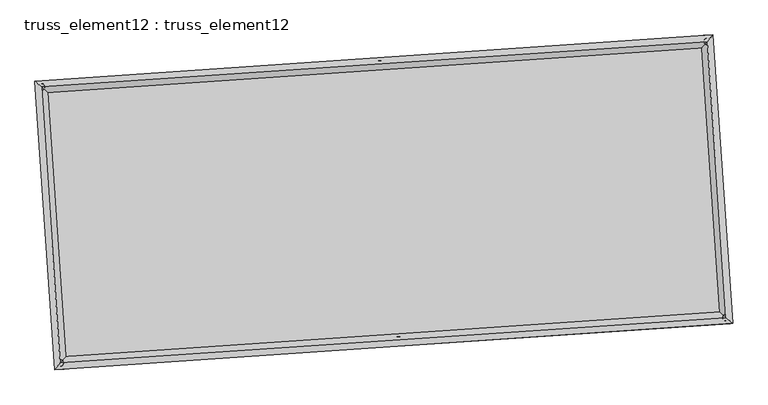
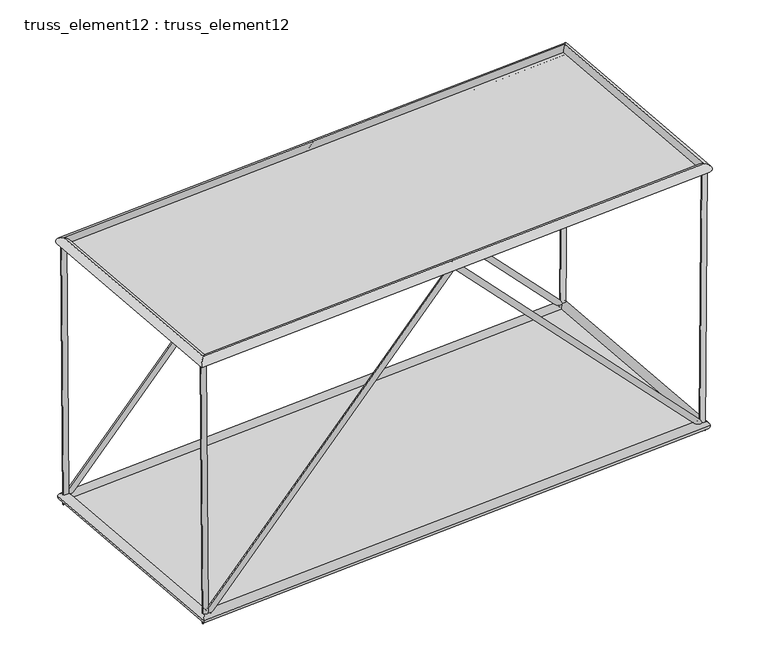
"""IFC4 building model written with IfcOpenShell, lengths in millimetres: plate geometry, truss_element12 : truss_element12."""

from ifc_helpers import new_model, si_unit, frame, origin, origin_with_axes, place, context, project, spatial, polyline, circle_curve, ellipse_curve, outline, extrude, source, transform, mapped, element, save
from ifc_brep_helpers import plane_surface, cylinder_surface, advanced_brep


def truss_element12_truss_element12_81932074(model_context):
    return source(origin(), model_context, "Body", "SolidModel", [
        advanced_brep(
        [(-3702.688172, 2273.6501932, 5000.2343714), (-3801.788684, 2260.2891126, 4999.4793629), (-3665.8706913, 2276.1606372, 123.2387715), (-3763.1161915, 2262.9260429, -123.2387715), (1063.4172149, 2598.6328018, 5071.9820194), (1063.8699312, 2592.0598775, 4927.7362286), (5793.2948238, 2921.145176, 123.2430249), (5891.4661532, 2921.2353125, -123.2430249), (5829.5270694, 2923.6157151, 5000.2328852), (5929.5240788, 2923.8303377, 4999.4898764)],
        [
            (0, 1, circle_curve(frame((-3752.238428, 2266.9696529, 4999.8568672), z_axis=(-0.007548997314577087, -0.000514737430455595, 0.999971373432721), x_axis=(-0.13361086689497337, 0.9910337470163174, -0.0004985201818760374)), 50.0)),
            (1, 0, circle_curve(frame((-3752.238428, 2266.9696529, 4999.8568672), z_axis=(-0.007548997314577087, -0.000514737430455595, 0.999971373432721), x_axis=(-0.13361086689497337, 0.9910337470163174, -0.0004985201818760374)), 50.0)),
            (0, 2),
            (2, 3, ellipse_curve(frame((-3714.4934414, 2269.54334, 0.0), z_axis=(-0.9271929359308112, -0.06322176171080186, 0.36921033084975474), x_axis=(0.36835501674811216, 0.025116728343544507, 0.9293458622029878)), 132.8968359, 50.0)),
            (3, 1),
            (3, 2, ellipse_curve(frame((-3714.4934414, 2269.54334, 0.0), z_axis=(-0.9271929359308112, -0.06322176171080186, 0.36921033084975474), x_axis=(0.36835501674811216, 0.025116728343544507, 0.9293458622029878)), 132.8968359, 50.0)),
            (2, 4),
            (4, 5, ellipse_curve(frame((1063.6435731, 2595.3463397, 4999.859124), z_axis=(-0.9976833955843888, -0.06802823819525586, -3.135687396447292e-05), x_axis=(3.12842325072798e-05, 2.133152891987861e-06, -0.9999999995083733)), 72.2799434, 50.0)),
            (5, 3),
            (5, 4, ellipse_curve(frame((1063.6435731, 2595.3463397, 4999.859124), z_axis=(-0.9976833955843888, -0.06802823819525586, -3.135687396447292e-05), x_axis=(3.12842325072798e-05, 2.133152891987861e-06, -0.9999999995083733)), 72.2799434, 50.0)),
            (4, 6),
            (6, 7, ellipse_curve(frame((5842.3804885, 2921.1902443, 0.0), z_axis=(-0.9271592320010842, -0.06321946356795421, -0.36929535326258833), x_axis=(-0.36843984219769044, -0.025122512268499313, 0.9293120800133075)), 132.9062538, 50.0)),
            (7, 5),
            (7, 6, ellipse_curve(frame((5842.3804885, 2921.1902443, 0.0), z_axis=(-0.9271592320010842, -0.06321946356795421, -0.36929535326258833), x_axis=(-0.36843984219769044, -0.025122512268499313, 0.9293120800133075)), 132.9062538, 50.0)),
            (8, 9, circle_curve(frame((5879.5255741, 2923.7230264, 4999.8613808), z_axis=(0.007429017120522426, 0.0005065564371105527, 0.9999722761682942), x_axis=(-0.0021499302803911083, 0.999997568554261, -0.0004905969378120464)), 50.0)),
            (9, 8, circle_curve(frame((5879.5255741, 2923.7230264, 4999.8613808), z_axis=(0.007429017120522426, 0.0005065564371105527, 0.9999722761682942), x_axis=(-0.0021499302803911083, 0.999997568554261, -0.0004905969378120464)), 50.0)),
            (6, 8),
            (9, 7),
        ],
        [
            plane_surface(frame((-3752.238428, 2316.9696463, 4999.8826048), z_axis=(-0.007548997314575647, -0.0005147374304560255, 0.9999713734327211), x_axis=(0.9999715059138159, -3.885862204455747e-06, 0.007548996314447718))),
            cylinder_surface(frame((-3752.238428, 2266.9696529, 4999.8568672), z_axis=(-0.007548997314577087, -0.000514737430455595, 0.999971373432721), x_axis=(-0.13361086689497337, 0.9910337470163174, -0.0004985201818760374)), 50.0),
            cylinder_surface(frame((-3714.4934414, 2269.54334, 0.0), z_axis=(-0.6901297168790946, -0.04705732196532738, -0.7221541264368931), x_axis=(-0.02041156189161515, 0.9987523773136525, -0.04557474027871566)), 50.0),
            cylinder_surface(frame((1063.6435731, 2595.3463397, 4999.859124), z_axis=(-0.6901748995971223, -0.04706040280311382, 0.7221107438988223), x_axis=(-0.115346442987764, 0.9922791286529746, -0.04557772405203943)), 50.0),
            plane_surface(frame((5879.5255741, 2873.7230329, 4999.8867094), z_axis=(0.007429017120522355, 0.0005065564371127904, 0.9999722761682942), x_axis=(0.999972404471555, -3.7633202953912764e-06, -0.0074290161673289294))),
            cylinder_surface(frame((5842.3804885, 2921.1902443, 0.0), z_axis=(-0.007429017120522424, -0.0005065564371105526, -0.999972276168294), x_axis=(-0.0021499302803911083, 0.999997568554261, -0.0004905969378120464)), 50.0),
        ],
        [
            (0, [[1, 2]]),
            (1, [[-1, 3, 4, 5]]),
            (1, [[-2, -5, 6, -3]]),
            (2, [[-4, 7, 8, 9]]),
            (2, [[-6, -9, 10, -7]]),
            (3, [[-8, 11, 12, 13]]),
            (3, [[-10, -13, 14, -11]]),
            (4, [[15, 16]]),
            (5, [[-12, 17, -16, 18]]),
            (5, [[-14, -18, -15, -17]]),
        ],
    ),
        advanced_brep(
        [(-3430.575219, -1717.0833911, 5000.2343714), (-3529.6757311, -1730.4444717, 4999.4793629), (-3393.7577384, -1714.5729471, 123.2387715), (-3491.0032386, -1727.8075414, -123.2387715), (1335.5301678, -1392.1007825, 5071.9820194), (1335.9828841, -1398.6737068, 4927.7362286), (6065.4077767, -1069.5884083, 123.2430249), (6163.5791061, -1069.4982718, -123.2430249), (6101.6400224, -1067.1178692, 5000.2328852), (6201.6370317, -1066.9032466, 4999.4898764)],
        [
            (0, 1, circle_curve(frame((-3480.1254751, -1723.7639314, 4999.8568672), z_axis=(-0.00754899731457709, -0.0005147374304555873, 0.999971373432721), x_axis=(-0.13361086689497323, 0.9910337470163173, -0.0004985201818760446)), 50.0)),
            (1, 0, circle_curve(frame((-3480.1254751, -1723.7639314, 4999.8568672), z_axis=(-0.00754899731457709, -0.0005147374304555873, 0.999971373432721), x_axis=(-0.13361086689497323, 0.9910337470163173, -0.0004985201818760446)), 50.0)),
            (0, 2),
            (2, 3, ellipse_curve(frame((-3442.3804885, -1721.1902443, 0.0), z_axis=(-0.9271929359308112, -0.06322176171080175, 0.3692103308497547), x_axis=(0.3683550167481121, 0.025116728343544472, 0.9293458622029878)), 132.8968359, 50.0)),
            (3, 1),
            (3, 2, ellipse_curve(frame((-3442.3804885, -1721.1902443, 0.0), z_axis=(-0.9271929359308112, -0.06322176171080175, 0.3692103308497547), x_axis=(0.3683550167481121, 0.025116728343544472, 0.9293458622029878)), 132.8968359, 50.0)),
            (2, 4),
            (4, 5, ellipse_curve(frame((1335.756526, -1395.3872446, 4999.859124), z_axis=(-0.9976833955843888, -0.06802823819525583, -3.135687396431242e-05), x_axis=(3.1284232507126054e-05, 2.1331528920551236e-06, -0.9999999995083733)), 72.2799434, 50.0)),
            (5, 3),
            (5, 4, ellipse_curve(frame((1335.756526, -1395.3872446, 4999.859124), z_axis=(-0.9976833955843888, -0.06802823819525583, -3.135687396431242e-05), x_axis=(3.1284232507126054e-05, 2.1331528920551236e-06, -0.9999999995083733)), 72.2799434, 50.0)),
            (4, 6),
            (6, 7, ellipse_curve(frame((6114.4934414, -1069.54334, 0.0), z_axis=(-0.9271592320010842, -0.06321946356795434, -0.3692953532625882), x_axis=(-0.3684398421976903, -0.025122512268499313, 0.9293120800133076)), 132.9062538, 50.0)),
            (7, 5),
            (7, 6, ellipse_curve(frame((6114.4934414, -1069.54334, 0.0), z_axis=(-0.9271592320010842, -0.06321946356795434, -0.3692953532625882), x_axis=(-0.3684398421976903, -0.025122512268499313, 0.9293120800133076)), 132.9062538, 50.0)),
            (8, 9, circle_curve(frame((6151.638527, -1067.0105579, 4999.8613808), z_axis=(0.0074290171205225845, 0.0005065564371106023, 0.9999722761682942), x_axis=(-0.002149930280391232, 0.999997568554261, -0.0004905969378120946)), 50.0)),
            (9, 8, circle_curve(frame((6151.638527, -1067.0105579, 4999.8613808), z_axis=(0.0074290171205225845, 0.0005065564371106023, 0.9999722761682942), x_axis=(-0.002149930280391232, 0.999997568554261, -0.0004905969378120946)), 50.0)),
            (6, 8),
            (9, 7),
        ],
        [
            plane_surface(frame((-3480.1254751, -1673.763938, 4999.8826048), z_axis=(-0.007548997314575647, -0.0005147374304560255, 0.9999713734327211), x_axis=(0.9999715059138159, -3.885862204455747e-06, 0.007548996314447718))),
            cylinder_surface(frame((-3480.1254751, -1723.7639314, 4999.8568672), z_axis=(-0.00754899731457709, -0.0005147374304555873, 0.999971373432721), x_axis=(-0.13361086689497323, 0.9910337470163173, -0.0004985201818760446)), 50.0),
            cylinder_surface(frame((-3442.3804885, -1721.1902443, 0.0), z_axis=(-0.6901297168790949, -0.047057321965327324, -0.722154126436893), x_axis=(-0.020411561891615058, 0.9987523773136525, -0.04557474027871568)), 50.0),
            cylinder_surface(frame((1335.756526, -1395.3872446, 4999.859124), z_axis=(-0.6901748995971222, -0.04706040280311387, 0.7221107438988226), x_axis=(-0.11534644298776417, 0.9922791286529747, -0.04557772405203947)), 50.0),
            plane_surface(frame((6151.638527, -1117.0105514, 4999.8867094), z_axis=(0.007429017120522355, 0.0005065564371127918, 0.9999722761682942), x_axis=(0.999972404471555, -3.763320294503098e-06, -0.0074290161673289294))),
            cylinder_surface(frame((6114.4934414, -1069.54334, 0.0), z_axis=(-0.007429017120522583, -0.0005065564371106022, -0.999972276168294), x_axis=(-0.002149930280391232, 0.999997568554261, -0.0004905969378120946)), 50.0),
        ],
        [
            (0, [[1, 2]]),
            (1, [[-1, 3, 4, 5]]),
            (1, [[-2, -5, 6, -3]]),
            (2, [[-4, 7, 8, 9]]),
            (2, [[-6, -9, 10, -7]]),
            (3, [[-8, 11, 12, 13]]),
            (3, [[-10, -13, 14, -11]]),
            (4, [[15, 16]]),
            (5, [[-12, 17, -16, 18]]),
            (5, [[-14, -18, -15, -17]]),
        ],
    ),
        advanced_brep(
        [(-3480.1242844, -1723.7626117, 4909.8568672), (-3480.1266658, -1723.7652511, 5089.8568672), (-3752.2397868, 2266.9707988, 5089.8568672), (-3752.2370692, 2266.968507, 4909.8568672), (5879.5266809, 2923.7243404, 5089.8613808), (5879.5244674, 2923.7217124, 4909.8613808), (6151.6398019, -1067.0117095, 5089.8613808), (6151.6372521, -1067.0094063, 4909.8613808)],
        [
            (0, 1, ellipse_curve(frame((-3480.1254751, -1723.7639314, 4999.8568672), z_axis=(-0.7535719234053797, 0.6573654662780873, -3.3059971506810466e-07), x_axis=(-0.657365466278005, -0.7535719234054516, -3.305997150681247e-07)), 127.2792206, 90.0)),
            (1, 2),
            (2, 3, ellipse_curve(frame((-3752.238428, 2266.9696529, 4999.8568672), z_axis=(-0.657365466278005, -0.7535719234054515, -3.3059971506814293e-07), x_axis=(0.7535719234053796, -0.6573654662780875, 3.3059971506812287e-07)), 127.2792206, 90.0)),
            (3, 0),
            (1, 0, ellipse_curve(frame((-3480.1254751, -1723.7639314, 4999.8568672), z_axis=(-0.7535719234053797, 0.6573654662780873, -3.3059971506810466e-07), x_axis=(-0.657365466278005, -0.7535719234054516, -3.305997150681247e-07)), 127.2792206, 90.0)),
            (3, 2, ellipse_curve(frame((-3752.238428, 2266.9696529, 4999.8568672), z_axis=(-0.657365466278005, -0.7535719234054515, -3.3059971506814293e-07), x_axis=(0.7535719234053796, -0.6573654662780875, 3.3059971506812287e-07)), 127.2792206, 90.0)),
            (2, 4),
            (4, 5, ellipse_curve(frame((5879.5255741, 2923.7230264, 4999.8613808), z_axis=(-0.7535719234053798, 0.6573654662780873, -3.3059971506814087e-07), x_axis=(-0.657365466278005, -0.7535719234054515, -3.30599715068125e-07)), 127.2792206, 90.0)),
            (5, 3),
            (5, 4, ellipse_curve(frame((5879.5255741, 2923.7230264, 4999.8613808), z_axis=(-0.7535719234053798, 0.6573654662780873, -3.3059971506814087e-07), x_axis=(-0.657365466278005, -0.7535719234054515, -3.30599715068125e-07)), 127.2792206, 90.0)),
            (4, 6),
            (6, 7, ellipse_curve(frame((6151.638527, -1067.0105579, 4999.8613808), z_axis=(0.657365466278005, 0.7535719234054516, 3.305997150681068e-07), x_axis=(-0.7535719234053797, 0.6573654662780875, -3.305997150681227e-07)), 127.2792206, 90.0)),
            (7, 5),
            (7, 6, ellipse_curve(frame((6151.638527, -1067.0105579, 4999.8613808), z_axis=(0.657365466278005, 0.7535719234054516, 3.305997150681068e-07), x_axis=(-0.7535719234053797, 0.6573654662780875, -3.305997150681227e-07)), 127.2792206, 90.0)),
            (6, 1),
            (0, 7),
        ],
        [
            cylinder_surface(frame((-3480.1254751, -1723.7639314, 4999.8568672), z_axis=(0.06802823822870085, -0.9976833960748767, 0.0), x_axis=(-0.9976833959743321, -0.0680282382218451, -1.4197044524281848e-05)), 90.0),
            cylinder_surface(frame((-3752.238428, 2266.9696529, 4999.8568672), z_axis=(-0.9976833960747679, -0.0680282382286909, -4.675386007660345e-07), x_axis=(-0.0680282382158825, 0.9976833959812822, -1.3729505923559892e-05)), 90.0),
            cylinder_surface(frame((5879.5255741, 2923.7230264, 4999.8613808), z_axis=(-0.0680282382287009, 0.9976833960748767, 0.0), x_axis=(0.9976833959871405, 0.0680282382227185, -1.3261967322837937e-05)), 90.0),
            cylinder_surface(frame((6151.638527, -1067.0105579, 4999.8613808), z_axis=(0.9976833960747677, 0.06802823822869078, 4.675386007660087e-07), x_axis=(0.06802823822869078, -0.9976833959804088, -1.3729505923559892e-05)), 90.0),
        ],
        [
            (0, [[1, 2, 3, 4]]),
            (0, [[5, -4, 6, -2]]),
            (1, [[-3, 7, 8, 9]]),
            (1, [[-6, -9, 10, -7]]),
            (2, [[-8, 11, 12, 13]]),
            (2, [[-10, -13, 14, -11]]),
            (3, [[-12, 15, -1, 16]]),
            (3, [[-14, -16, -5, -15]]),
        ],
    ),
        advanced_brep(
        [(-3358.7115243, -1625.2761972, 0.0), (-3526.0494527, -1817.1042913, 0.0), (-3810.4074885, 2353.2123043, 0.0), (-3618.5793943, 2185.8743758, 0.0), (5926.0494527, 3017.1042913, 0.0), (5758.7115243, 2825.2761972, 0.0), (6210.4074885, -1153.2123043, 0.0), (6018.5793943, -985.8743758, 0.0)],
        [
            (0, 1, ellipse_curve(frame((-3442.3804885, -1721.1902443, 0.0), z_axis=(-0.7535719234054581, 0.6573654662780807, 0.0), x_axis=(-0.6573654662780808, -0.7535719234054581, 0.0)), 127.2792206, 90.0)),
            (1, 2),
            (2, 3, ellipse_curve(frame((-3714.4934414, 2269.54334, 0.0), z_axis=(-0.6573654662780807, -0.753571923405458, 0.0), x_axis=(0.7535719234054579, -0.6573654662780808, 0.0)), 127.2792206, 90.0)),
            (3, 0),
            (1, 0, ellipse_curve(frame((-3442.3804885, -1721.1902443, 0.0), z_axis=(-0.7535719234054581, 0.6573654662780807, 0.0), x_axis=(-0.6573654662780808, -0.7535719234054581, 0.0)), 127.2792206, 90.0)),
            (3, 2, ellipse_curve(frame((-3714.4934414, 2269.54334, 0.0), z_axis=(-0.6573654662780807, -0.753571923405458, 0.0), x_axis=(0.7535719234054579, -0.6573654662780808, 0.0)), 127.2792206, 90.0)),
            (2, 4),
            (4, 5, ellipse_curve(frame((5842.3804885, 2921.1902443, 0.0), z_axis=(-0.7535719234054582, 0.6573654662780806, 0.0), x_axis=(-0.6573654662780805, -0.7535719234054583, 0.0)), 127.2792206, 90.0)),
            (5, 3),
            (5, 4, ellipse_curve(frame((5842.3804885, 2921.1902443, 0.0), z_axis=(-0.7535719234054582, 0.6573654662780806, 0.0), x_axis=(-0.6573654662780805, -0.7535719234054583, 0.0)), 127.2792206, 90.0)),
            (4, 6),
            (6, 7, ellipse_curve(frame((6114.4934414, -1069.54334, 0.0), z_axis=(0.6573654662780806, 0.7535719234054581, 0.0), x_axis=(-0.7535719234054581, 0.6573654662780806, 0.0)), 127.2792206, 90.0)),
            (7, 5),
            (7, 6, ellipse_curve(frame((6114.4934414, -1069.54334, 0.0), z_axis=(0.6573654662780806, 0.7535719234054581, 0.0), x_axis=(-0.7535719234054581, 0.6573654662780806, 0.0)), 127.2792206, 90.0)),
            (6, 1),
            (0, 7),
        ],
        [
            cylinder_surface(frame((-3442.3804885, -1721.1902443, 0.0), z_axis=(0.06802823822870274, -0.9976833960748764, 0.0), x_axis=(-0.9976833960748764, -0.06802823822870274, 0.0)), 90.0),
            cylinder_surface(frame((-3714.4934414, 2269.54334, 0.0), z_axis=(-0.9976833960748767, -0.06802823822870008, 0.0), x_axis=(-0.06802823822870008, 0.9976833960748767, 0.0)), 90.0),
            cylinder_surface(frame((5842.3804885, 2921.1902443, 0.0), z_axis=(-0.06802823822870283, 0.9976833960748764, 0.0), x_axis=(0.9976833960748764, 0.06802823822870283, 0.0)), 90.0),
            cylinder_surface(frame((6114.4934414, -1069.54334, 0.0), z_axis=(0.9976833960748767, 0.06802823822870016, 0.0), x_axis=(0.06802823822870016, -0.9976833960748767, 0.0)), 90.0),
        ],
        [
            (0, [[1, 2, 3, 4]]),
            (0, [[5, -4, 6, -2]]),
            (1, [[-3, 7, 8, 9]]),
            (1, [[-6, -9, 10, -7]]),
            (2, [[-8, 11, 12, 13]]),
            (2, [[-10, -13, 14, -11]]),
            (3, [[-12, 15, -1, 16]]),
            (3, [[-14, -16, -5, -15]]),
        ],
    ),
        extrude(outline(polyline([(-3442.3804885, -1721.1902443), (-3714.4934414, 2269.54334), (5842.3804885, 2921.1902443), (6114.4934414, -1069.54334), (-3442.3804885, -1721.1902443)])), origin_with_axes(), (0.0, 0.0, 1.0), 20.0),
        extrude(outline(polyline([(-2000.0, 4827.0643974), (2000.0, 4827.0643974), (2000.0, -4827.0643974), (-2000.0, -4827.0643974), (-2000.0, 4827.0643974)])), frame((1199.7000495, 599.9795475, 4999.859124), z_axis=(-4.6645549900834067e-07, -3.180582731402529e-08, 0.9999999999998909), x_axis=(-0.06802823822870274, 0.9976833960748764, 0.0)), (0.0, 0.0, 1.0), 20.0),
    ])


if __name__ == "__main__":
    model = new_model("IFC4")
    model_context = context("Model", 3, world=origin())
    ifc_project = project(units=[si_unit("LENGTHUNIT", "METRE", prefix="MILLI")], contexts=[model_context])
    site = spatial("IfcSite", under=ifc_project)
    building = spatial("IfcBuilding", under=site)
    placement = place(None, origin())
    truss_element12_truss_element12_shape = truss_element12_truss_element12_81932074(model_context)
    element("IfcPlate", 1, ObjectType="truss_element12 : truss_element12", at=placement, inside=building, context=model_context, shape_type="MappedRepresentation", body=[
        mapped(truss_element12_truss_element12_shape, transform((0.0, 0.0, 0.0), x_axis=(1.0, 0.0, 0.0), y_axis=(0.0, 1.0, 0.0), z_axis=(0.0, 0.0, 1.0))),
    ])
    save(model, "model.ifc")

# Revit data of these elements
# Type "truss_element12 : truss_element12"
#   steellbar1 = 90 mm
#   steelbar2 = 50 mm
#   offset1 = 5000 mm
#   M = Default Roof
# Element 1 (IfcPlate, "truss_element12 : truss_element12")
#   Materials on its faces: "Default Roof"
# Materials
#   "Default Roof": class "Miscellaneous", colour RGB 0 127 0, transparency 0, Comments = "Rendering appearance not upgraded Rendering appearance not upgraded ", Cost = 0
